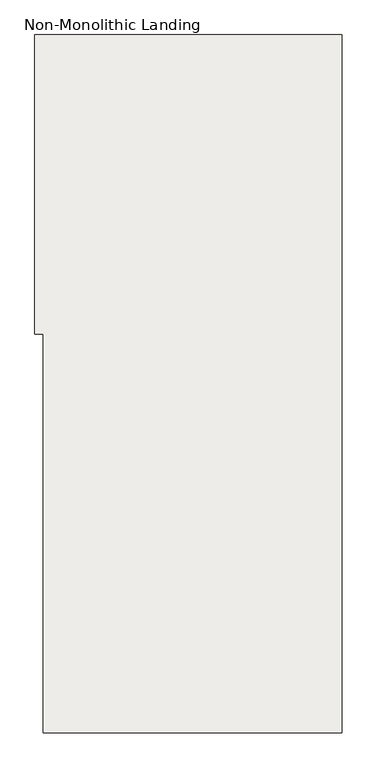
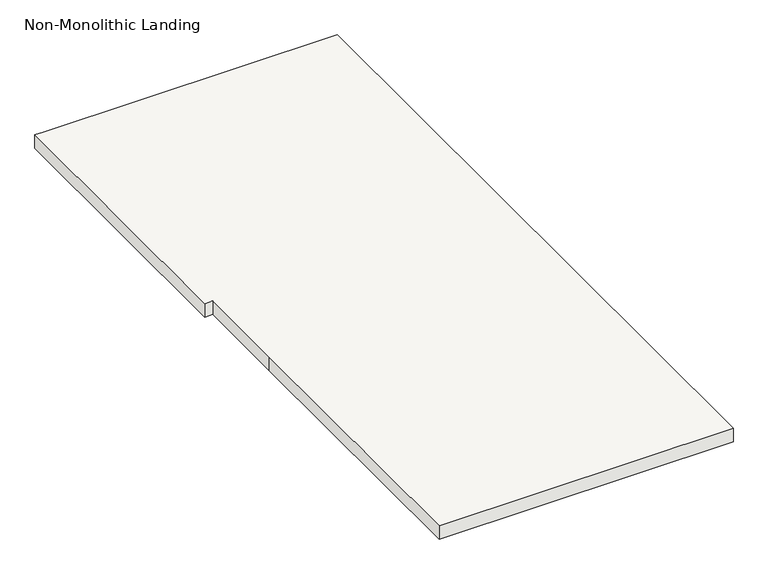
"""IFC4 building model written with IfcOpenShell, lengths in millimetres: slab geometry, Non-Monolithic Landing."""

import ifcopenshell
import ifcopenshell.guid

model = None  # the IFC model being written
_history = None  # IfcOwnerHistory: only IFC2X3 demands one
_inside = {}  # id of a spatial element -> (the spatial element, [elements in it])
_under = {}  # id of a project, library or spatial element -> (it, [spatial elements below it])
_declared = {}  # id of a project -> (the project, [libraries it declares])
_typed = {}  # id of a type object -> (the type object, [elements of that type])
_made_of = {}  # id of a material, layer set ... -> (it, [elements and type objects made of it])


def new_model(schema):
    """Start an empty IFC model of exactly this schema.

    Asked for "IFC4X3", IfcOpenShell would pick the latest addendum, in which some entities
    have other attributes; the version numbers below select the first issue.
    IFC2X3 requires an IfcOwnerHistory on every rooted entity: one is made here for all.
    """
    global model, _history
    if schema == "IFC4X3":
        model = ifcopenshell.file(schema_version=(4, 3, 0, 0))
    else:
        model = ifcopenshell.file(schema=schema)
    _inside.clear()
    _under.clear()
    _declared.clear()
    _typed.clear()
    _made_of.clear()
    _history = None
    if model.schema == "IFC2X3":
        org = make("IfcOrganization", Name="unknown")
        user = make(
            "IfcPersonAndOrganization",
            ThePerson=make("IfcPerson", FamilyName="unknown"),
            TheOrganization=org,
        )
        app = make(
            "IfcApplication",
            ApplicationDeveloper=org,
            Version="unknown",
            ApplicationFullName="unknown",
            ApplicationIdentifier="unknown",
        )
        _history = make(
            "IfcOwnerHistory",
            OwningUser=user,
            OwningApplication=app,
            ChangeAction="ADDED",
            CreationDate=0,
        )
    return model


def make(cls, **values):
    """One entity of the class cls with the attributes given. An attribute that is None is left unset."""
    return model.create_entity(
        cls, **{name: value for name, value in values.items() if value is not None}
    )


def rooted(cls, **values):
    """An entity with a GlobalId (a new one), such as an element, a storey or a relation."""
    return make(cls, GlobalId=ifcopenshell.guid.new(), OwnerHistory=_history, **values)


def si_unit(unit_type, name, prefix=None):
    """IfcSIUnit, for example si_unit("LENGTHUNIT", "METRE", prefix="MILLI")."""
    return make("IfcSIUnit", UnitType=unit_type, Prefix=prefix, Name=name)


def assignment(units):
    """IfcUnitAssignment: the units of a project."""
    return None if units is None else make("IfcUnitAssignment", Units=units)


def point(xyz):
    """IfcCartesianPoint."""
    return None if xyz is None else make("IfcCartesianPoint", Coordinates=xyz)


def direction(xyz):
    """IfcDirection."""
    return None if xyz is None else make("IfcDirection", DirectionRatios=xyz)


def frame(location, z_axis=None, x_axis=None):
    """IfcAxis2Placement3D, a coordinate frame: its origin and axes. An axis left out is left unset."""
    return make(
        "IfcAxis2Placement3D",
        Location=point(location),
        Axis=direction(z_axis),
        RefDirection=direction(x_axis),
    )


def origin():
    """The frame at (0, 0, 0) with its axes left unset."""
    return frame((0.0, 0.0, 0.0))


def place(relative_to, where):
    """IfcLocalPlacement: puts the frame where relative to a parent placement (None: the world)."""
    return make(
        "IfcLocalPlacement", PlacementRelTo=relative_to, RelativePlacement=where
    )


def context(
    kind, dimensions, precision=None, world=None, true_north=None, identifier=None
):
    """IfcGeometricRepresentationContext, for example the 3D "Model" context."""
    return make(
        "IfcGeometricRepresentationContext",
        ContextIdentifier=identifier,
        ContextType=kind,
        CoordinateSpaceDimension=dimensions,
        Precision=precision,
        WorldCoordinateSystem=world,
        TrueNorth=true_north,
    )


def project(units=None, contexts=None):
    """IfcProject with its units and contexts."""
    return rooted(
        "IfcProject",
        Name="project",
        RepresentationContexts=contexts,
        UnitsInContext=assignment(units),
    )


def spatial(cls, under=None, at=None, **own):
    """A site, building, storey or space (cls), placed at a placement, below another one or the project."""
    s = rooted(cls, ObjectPlacement=at, **own)
    if under is not None:
        _under.setdefault(under.id(), (under, []))[1].append(s)
    return s


def polyline(points):
    """IfcPolyline through the points."""
    return make("IfcPolyline", Points=[point(p) for p in points])


def outline(outer, holes=None, kind="AREA"):
    """IfcArbitraryClosedProfileDef: a profile drawn as a closed curve; with holes, ...WithVoids."""
    if holes is None:
        return make("IfcArbitraryClosedProfileDef", ProfileType=kind, OuterCurve=outer)
    return make(
        "IfcArbitraryProfileDefWithVoids",
        ProfileType=kind,
        OuterCurve=outer,
        InnerCurves=holes,
    )


def extrude(swept, where, along, depth):
    """IfcExtrudedAreaSolid: the profile swept, set in the frame where, extruded along a direction by depth."""
    return make(
        "IfcExtrudedAreaSolid",
        SweptArea=swept,
        Position=where,
        ExtrudedDirection=direction(along),
        Depth=depth,
    )


def shape(context_of_items, identifier, shape_type, items):
    """IfcShapeRepresentation: the items that make up one representation, for example the "Body"."""
    return make(
        "IfcShapeRepresentation",
        ContextOfItems=context_of_items,
        RepresentationIdentifier=identifier,
        RepresentationType=shape_type,
        Items=items,
    )


def source(mapping_origin, context_of_items, identifier, shape_type, items):
    """IfcRepresentationMap: a shape defined once, which mapped items show again and again."""
    return make(
        "IfcRepresentationMap",
        MappingOrigin=mapping_origin,
        MappedRepresentation=shape(context_of_items, identifier, shape_type, items),
    )


def transform(
    local_origin,
    x_axis=None,
    y_axis=None,
    z_axis=None,
    scale=None,
    scale2=None,
    scale3=None,
    uniform=True,
):
    """IfcCartesianTransformationOperator3D, or its non-uniform kind. x_axis, y_axis, z_axis: its Axis1, 2, 3."""
    if uniform:
        return make(
            "IfcCartesianTransformationOperator3D",
            Axis1=direction(x_axis),
            Axis2=direction(y_axis),
            LocalOrigin=point(local_origin),
            Scale=scale,
            Axis3=direction(z_axis),
        )
    return make(
        "IfcCartesianTransformationOperator3DnonUniform",
        Axis1=direction(x_axis),
        Axis2=direction(y_axis),
        LocalOrigin=point(local_origin),
        Scale=scale,
        Axis3=direction(z_axis),
        Scale2=scale2,
        Scale3=scale3,
    )


def mapped(mapping_source, mapping_target):
    """IfcMappedItem: shows the shape of a source again, moved by a transform."""
    return make(
        "IfcMappedItem", MappingSource=mapping_source, MappingTarget=mapping_target
    )


def made_of(thing, what):
    """Note that an element or type object is made of a material, layer set ...; save() writes the relation."""
    if what is not None:
        _made_of.setdefault(what.id(), (what, []))[1].append(thing)
    return thing


def element(
    cls,
    number,
    at=None,
    inside=None,
    cuts=None,
    type_object=None,
    material=None,
    context=None,
    identifier="Body",
    shape_type=None,
    held_by="IfcProductDefinitionShape",
    body=None,
    shapes=None,
    **own,
):
    """One element of the class cls, such as IfcWall. Its Tag is "e" and its number.

    at: its placement. inside: the storey or other place that contains it. cuts: it is an
    opening in that element (IfcRelVoidsElement). A single representation is given by context,
    identifier, shape_type and body (its items); several are given by shapes. held_by: the class
    of the entity that holds the representations. save() writes the other relations.
    """
    e = rooted(cls, Tag="e%d" % number, ObjectPlacement=at, **own)
    if body is not None:
        shapes = [shape(context, identifier, shape_type, body)]
    if shapes is not None:
        e.Representation = make(held_by, Representations=shapes)
    if inside is not None:
        _inside.setdefault(inside.id(), (inside, []))[1].append(e)
    if cuts is not None:
        rooted(
            "IfcRelVoidsElement", RelatingBuildingElement=cuts, RelatedOpeningElement=e
        )
    if type_object is not None:
        _typed.setdefault(type_object.id(), (type_object, []))[1].append(e)
    return made_of(e, material)


def aggregate(whole, parts):
    """IfcRelAggregates: a whole, such as a stair, and the parts it consists of."""
    return rooted("IfcRelAggregates", RelatingObject=whole, RelatedObjects=parts)


def save(model, path):
    """Write the relations noted so far, then the file.

    IfcRelAggregates (storeys below a building ...), IfcRelContainedInSpatialStructure (elements
    in a storey), IfcRelDefinesByType, IfcRelAssociatesMaterial and IfcRelDeclares: one each for
    every whole, place, type object, material and project.
    """
    for whole, parts in _under.values():
        aggregate(whole, parts)
    for where, things in _inside.values():
        rooted(
            "IfcRelContainedInSpatialStructure",
            RelatedElements=things,
            RelatingStructure=where,
        )
    for kind, things in _typed.values():
        rooted("IfcRelDefinesByType", RelatedObjects=things, RelatingType=kind)
    for what, things in _made_of.values():
        rooted("IfcRelAssociatesMaterial", RelatedObjects=things, RelatingMaterial=what)
    for by, libraries in _declared.values():
        rooted("IfcRelDeclares", RelatingContext=by, RelatedDefinitions=libraries)
    model.write(path)


def non_monolithic_landing_c05d15c3(model_context):
    return source(origin(), model_context, "Body", "SweptSolid", [
        extrude(outline(polyline([(-16004.0481446, -4273.6871906), (-16004.0481446, -3968.8871906), (-16029.4481446, -3968.8871906), (-16029.4481446, -3054.4871906), (-16004.0481446, -3054.4871906), (-15089.6481446, -3054.4871906), (-15089.6481446, -5188.0871906), (-16004.0481446, -5188.0871906), (-16004.0481446, -4273.6871906)])), frame((0.0, 0.0, 1479.55), z_axis=(0.0, 0.0, 1.0), x_axis=(1.0, 0.0, 0.0)), (0.0, 0.0, 1.0), 44.45),
    ])


if __name__ == "__main__":
    model = new_model("IFC4")
    model_context = context("Model", 3, world=origin())
    ifc_project = project(units=[si_unit("LENGTHUNIT", "METRE", prefix="MILLI")], contexts=[model_context])
    site = spatial("IfcSite", under=ifc_project)
    building = spatial("IfcBuilding", under=site)
    placement = place(None, origin())
    non_monolithic_landing_shape = non_monolithic_landing_c05d15c3(model_context)
    element("IfcSlab", 1, ObjectType="Non-Monolithic Landing", at=placement, inside=building, context=model_context, shape_type="MappedRepresentation", body=[
        mapped(non_monolithic_landing_shape, transform((0.0, 0.0, 0.0), x_axis=(1.0, 0.0, 0.0), y_axis=(0.0, 1.0, 0.0), z_axis=(0.0, 0.0, 1.0))),
    ])
    save(model, "model.ifc")

# Revit data of these elements
# Element 1 (IfcSlab, "Non-Monolithic Landing")
#   Materials on its faces: "Wood - Flooring"
# Materials
#   "Wood - Flooring": class "Unassigned", colour RGB 216 169 114, transparency 0
